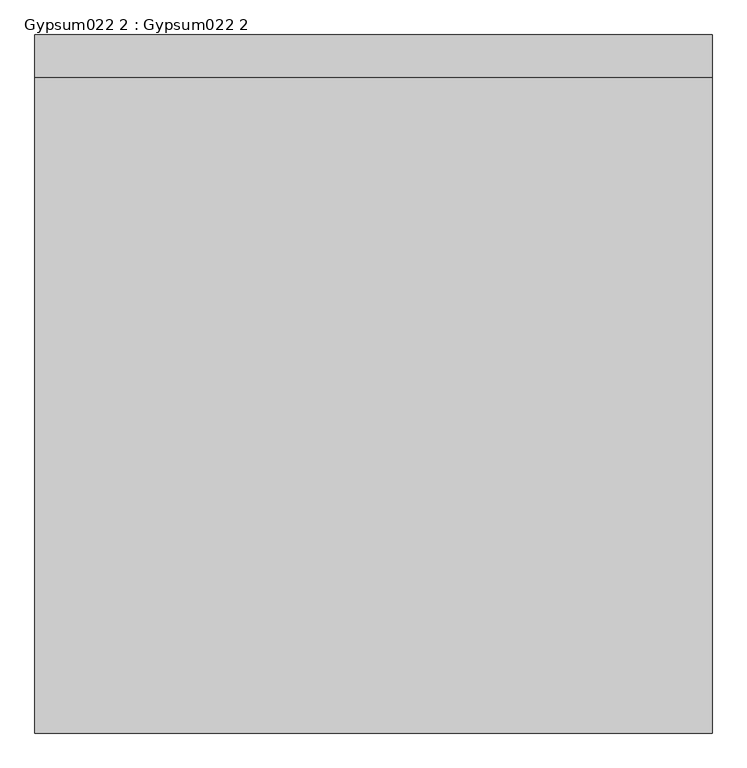
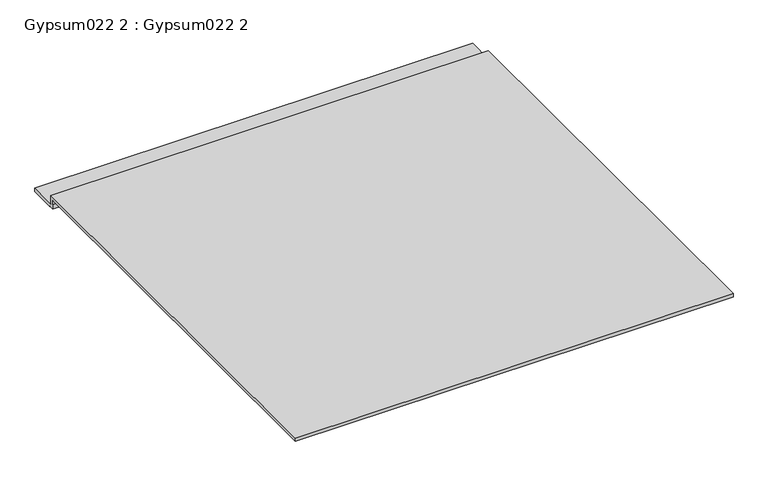
"""IFC4 building model written with IfcOpenShell, lengths in millimetres: proxy geometry, Gypsum022 2 : Gypsum022 2."""

from ifc_helpers import new_model, si_unit, frame, origin, place, context, project, spatial, polyline, outline, extrude, source, transform, mapped, element, save


def gypsum022_2_gypsum022_2_470ce31a(model_context):
    return source(origin(), model_context, "Body", "SweptSolid", [
        extrude(outline(polyline([(9592.4838724, 39569.7710938), (9592.4838724, 39528.496), (9718.4918386, 39528.496), (9718.4918386, 39512.621), (9599.0420564, 39512.621), (9599.0420564, 39513.901), (9577.8888724, 39513.901), (9577.8888724, 39535.0541839), (9576.6088724, 39535.0541839), (9576.6088724, 39553.8960938), (7656.2019482, 39553.8960938), (7656.2019482, 39569.7710938), (9592.4838724, 39569.7710938)])), frame((3694.0383192, 0.0, 0.0), z_axis=(1.0, 0.0, 0.0), x_axis=(0.0, 1.0, 0.0)), (0.0, 0.0, 1.0), 2000.25),
    ])


if __name__ == "__main__":
    model = new_model("IFC4")
    model_context = context("Model", 3, world=origin())
    ifc_project = project(units=[si_unit("LENGTHUNIT", "METRE", prefix="MILLI")], contexts=[model_context])
    site = spatial("IfcSite", under=ifc_project)
    building = spatial("IfcBuilding", under=site)
    placement = place(None, origin())
    gypsum022_2_gypsum022_2_shape = gypsum022_2_gypsum022_2_470ce31a(model_context)
    element("IfcBuildingElementProxy", 1, Name="Gypsum022 2 : Gypsum022 2", ObjectType="Gypsum022 2 : Gypsum022 2", at=placement, inside=building, context=model_context, shape_type="MappedRepresentation", body=[
        mapped(gypsum022_2_gypsum022_2_shape, transform((0.0, 0.0, 0.0), x_axis=(1.0, 0.0, 0.0), y_axis=(0.0, 1.0, 0.0), z_axis=(0.0, 0.0, 1.0))),
    ])
    save(model, "model.ifc")

# Revit data of these elements
# Type "Gypsum022 2 : Gypsum022 2"
#   NameOverride = "Gypsum022"
# Element 1 (IfcBuildingElementProxy, "Gypsum022 2 : Gypsum022 2")
#   Materials on its faces: "5/8\"  GYPSUM BOARD"
# Materials
#   "5/8\"  GYPSUM BOARD": class "Unassigned", colour RGB 255 255 255, transparency 0, Cost = 0
